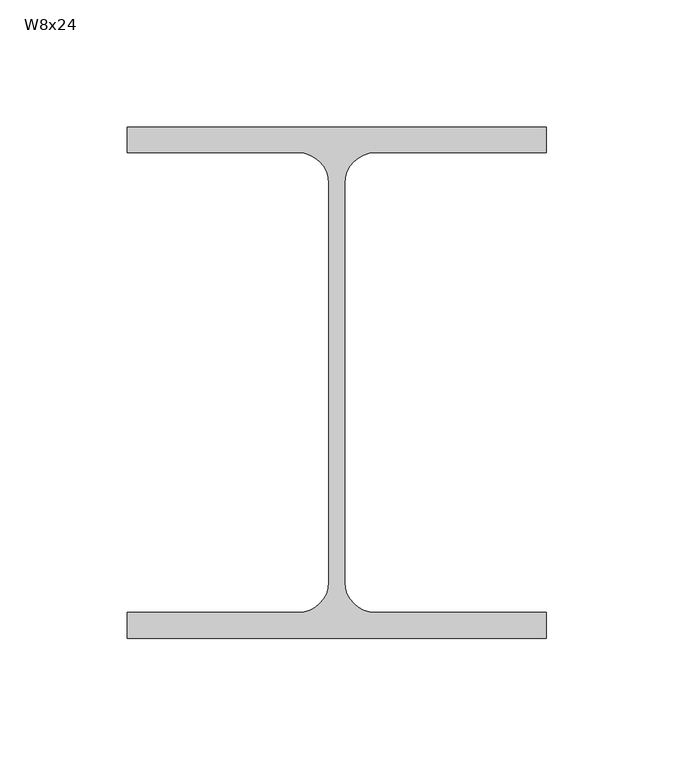
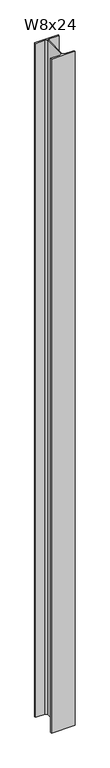
"""IFC4 building model written with IfcOpenShell, lengths in millimetres: column geometry, RME WF - Column : W8x24."""

from ifc_helpers import new_model, si_unit, point, frame, frame_2d, origin, place, context, project, spatial, polyline, circle_curve, trimmed, segment, composite_curve, outline, extrude, source, transform, mapped, element, save


def w8x24_99ef15d7(model_context):
    return source(origin(), model_context, "Body", "SweptSolid", [
        extrude(outline(composite_curve([segment(polyline([(82.55, 100.711), (82.55, 90.551), (15.1765, 90.551)]), True, "CONTINUOUS"), segment(trimmed(circle_curve(frame_2d((15.1765, 78.486)), 12.065), [point((15.1765, 90.551))], [point((3.1115, 78.486))], True, "CARTESIAN"), True, "CONTINUOUS"), segment(polyline([(3.1115, 78.486), (3.1115, -78.486)]), True, "CONTINUOUS"), segment(trimmed(circle_curve(frame_2d((15.1765, -78.486)), 12.065), [point((3.1115, -78.486))], [point((15.1765, -90.551))], True, "CARTESIAN"), True, "CONTINUOUS"), segment(polyline([(15.1765, -90.551), (82.55, -90.551), (82.55, -100.711), (-82.55, -100.711), (-82.55, -90.551), (-15.1765, -90.551)]), True, "CONTINUOUS"), segment(trimmed(circle_curve(frame_2d((-15.1765, -78.486)), 12.065), [point((-15.1765, -90.551))], [point((-3.1115, -78.486))], True, "CARTESIAN"), True, "CONTINUOUS"), segment(polyline([(-3.1115, -78.486), (-3.1115, 78.486)]), True, "CONTINUOUS"), segment(trimmed(circle_curve(frame_2d((-15.1765, 78.486)), 12.065), [point((-3.1115, 78.486))], [point((-15.1765, 90.551))], True, "CARTESIAN"), True, "CONTINUOUS"), segment(polyline([(-15.1765, 90.551), (-82.55, 90.551), (-82.55, 100.711), (82.55, 100.711)]), True, "CONTINUOUS")], self_intersect=False)), frame((0.0, 0.0, -304.8), z_axis=(0.0, 0.0, 1.0), x_axis=(1.0, 0.0, 0.0)), (0.0, 0.0, 1.0), 4978.4),
    ])


if __name__ == "__main__":
    model = new_model("IFC4")
    model_context = context("Model", 3, world=origin())
    ifc_project = project(units=[si_unit("LENGTHUNIT", "METRE", prefix="MILLI")], contexts=[model_context])
    site = spatial("IfcSite", under=ifc_project)
    building = spatial("IfcBuilding", under=site)
    placement = place(None, origin())
    w8x24_shape = w8x24_99ef15d7(model_context)
    element("IfcColumn", 1, ObjectType="RME WF - Column : W8x24", at=placement, inside=building, context=model_context, shape_type="MappedRepresentation", body=[
        mapped(w8x24_shape, transform((0.0, 0.0, 0.0), x_axis=(1.0, 0.0, 0.0), y_axis=(0.0, 1.0, 0.0), z_axis=(0.0, 0.0, 1.0))),
    ])
    save(model, "model.ifc")

# Revit data of these elements
# Type "RME WF - Column : W8x24"
#   Type Mark = "C1"
#   REINF TYPE [instance default] = ""
#   Nominal Size = "W16"
#   COL REMARKS [instance default] = ""
#   BP [instance default] = ""
#   Assembly Code = "B10"
#   W = 24
#   bf = 0' - 6 1/2"
#   d = 0' - 7.93"
#   k = 0' - 0 7/8"
#   kr = 0' - 0.475"
#   tf = 0' - 0.4"
#   tw = 0' - 0.245"
#   A = 0.0491667 SF
#   Structural Material [instance default] = Metal - Steel - ASTM A992
# Element 1 (IfcColumn, "RME WF - Column : W8x24")
#   Materials on its faces: "Metal - Steel - ASTM A992"
# Materials
#   "Metal - Steel - ASTM A992": class "Metal", colour RGB 255 128 0, transparency 0
